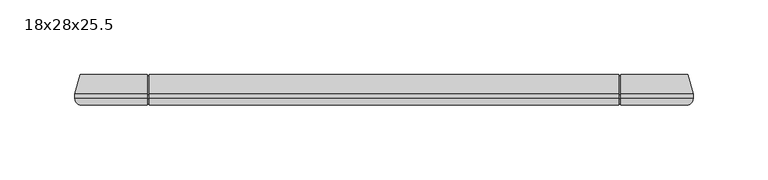
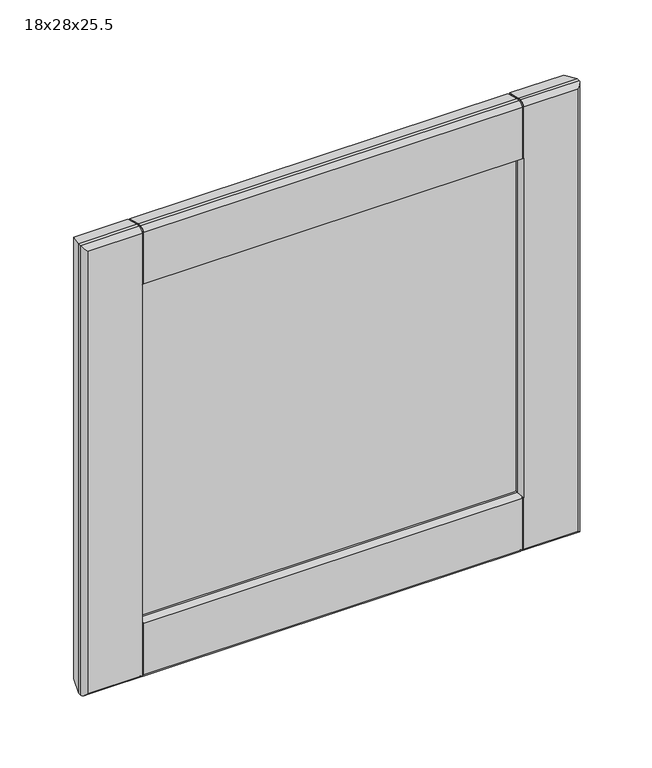
"""IFC4 building model written with IfcOpenShell, lengths in millimetres: furniture geometry, Cabinet-Base-Merillat-Peninsula_Single_Door-Marlin : 18x28x25.5."""

from ifc_helpers import new_model, si_unit, frame, origin, place, context, project, spatial, polyline, circle_curve, ellipse_curve, outline, extrude, source, transform, mapped, element, save
from ifc_brep_helpers import plane_surface, cylinder_surface, advanced_brep


def furniture_18x28x25_5_82de7a22(model_context):
    return source(origin(), model_context, "Body", "SolidModel", [
        advanced_brep(
        [(225.1127049, -696.09335, 63.5), (225.1127049, -696.09335, 457.2), (222.0162124, -700.56375, 454.1035075), (222.0162124, -700.56375, 66.5964925), (225.1127049, -693.32475, 63.5), (225.1127049, -693.32475, 457.2), (221.6075049, -680.24375, 67.0052), (221.6075049, -680.24375, 453.6948), (176.9115422, -680.24375, 111.7011628), (176.5414105, -681.0375, 112.0712945), (174.4602514, -685.50056, 114.1524535), (174.4602514, -685.50056, 406.5475465), (176.5414105, -681.0375, 408.6287055), (176.9115422, -680.24375, 408.9988372), (175.8600209, -687.7406593, 112.752684), (175.8600209, -687.7406593, 407.947316), (190.1877049, -687.99075, 98.425), (190.1877049, -687.99075, 422.275), (190.1877049, -692.81675, 98.425), (190.1877049, -692.81675, 422.275), (175.8600209, -693.0668407, 112.752684), (175.8600209, -693.0668407, 407.947316), (174.4602514, -695.30694, 114.1524535), (174.4602514, -695.30694, 406.5475465), (176.5414105, -699.77, 112.0712945), (176.9086747, -700.5576008, 111.7040302), (176.9115422, -700.56375, 408.9988372), (176.5414105, -699.77, 408.6287055), (-184.5408026, -700.56375, 454.1035075), (-139.4730764, -700.56375, 454.1035075), (-139.4730764, -696.09335, 457.2), (-187.6372951, -696.09335, 457.2), (176.9086747, -696.09335, 457.2), (176.9086747, -700.56375, 454.1035075), (175.3211747, -696.09335, 457.2), (-137.8855764, -696.09335, 457.2), (-137.8855764, -700.56375, 454.1035075), (175.3211747, -700.56375, 454.1035075), (-139.4730764, -693.32475, 457.2), (-187.6372951, -693.32475, 457.2), (176.9086747, -693.32475, 457.2), (175.3211747, -693.32475, 457.2), (-137.8855764, -693.32475, 457.2), (-139.4730764, -680.24375, 453.6948), (-184.1320951, -680.24375, 453.6948), (175.3211747, -680.24375, 453.6948), (-137.8855764, -680.24375, 453.6948), (176.9086747, -680.24375, 453.6948), (-136.9848416, -685.50056, 406.5475465), (-139.0660006, -681.0375, 408.6287055), (-137.8855764, -681.0375, 408.6287055), (-137.8855764, -680.24375, 408.9988372), (175.3211747, -680.24375, 408.9988372), (175.3211747, -681.0375, 408.6287055), (-138.384611, -687.7406593, 407.947316), (-152.7122951, -687.99075, 422.275), (-152.7122951, -692.81675, 422.275), (-138.384611, -693.0668407, 407.947316), (-136.9848416, -695.30694, 406.5475465), (175.3211747, -699.77, 408.6287055), (175.3211747, -700.56375, 408.9988372), (-137.8855764, -700.56375, 408.9988372), (-137.8855764, -699.77, 408.6287055), (-139.0660006, -699.77, 408.6287055), (-187.6372951, -696.09335, 63.5), (-184.5408026, -700.56375, 66.5964925), (-187.6372951, -693.32475, 63.5), (-184.1320951, -680.24375, 67.0052), (-139.4361323, -680.24375, 408.9988372), (-136.9848416, -685.50056, 114.1524535), (-139.0660006, -681.0375, 112.0712945), (-139.4361323, -680.24375, 111.7011628), (-138.384611, -687.7406593, 112.752684), (-152.7122951, -687.99075, 98.425), (-152.7122951, -692.81675, 98.425), (-138.384611, -693.0668407, 112.752684), (-136.9848416, -695.30694, 114.1524535), (-139.4361323, -700.56375, 408.9988372), (-139.4361323, -700.56375, 111.7011628), (-139.0660006, -699.77, 112.0712945), (176.9086747, -700.56375, 66.5964925), (176.9086747, -696.09335, 63.5), (-139.4730764, -696.09335, 63.5), (-139.4730764, -700.56375, 66.5964925), (-137.8855764, -696.09335, 63.5), (175.3211747, -696.09335, 63.5), (175.3211747, -700.56375, 66.5964925), (-137.8855764, -700.56375, 66.5964925), (176.9086747, -693.32475, 63.5), (-139.4730764, -693.32475, 63.5), (-137.8855764, -693.32475, 63.5), (175.3211747, -693.32475, 63.5), (176.9086747, -680.24375, 67.0052), (-139.4730764, -680.24375, 67.0052), (-137.8855764, -680.24375, 67.0052), (175.3211747, -680.24375, 67.0052), (-137.8855764, -680.24375, 111.7011628), (175.3211747, -680.24375, 111.7011628), (175.3211747, -681.0375, 112.0712945), (-137.8855764, -681.0375, 112.0712945), (-137.8855764, -699.77, 112.0712945), (-137.8855764, -700.56375, 111.7011628), (175.3211747, -700.56375, 111.7011628), (175.3211747, -699.77, 112.0712945), (-137.8855764, -699.77, 66.7473948), (-137.8855764, -696.09335, 64.29375), (-137.8855764, -693.4292537, 64.29375), (-137.8855764, -681.0375, 67.6142588), (-139.4730764, -681.0375, 112.0712945), (-139.4730764, -681.0375, 67.6142588), (-139.4730764, -693.4292537, 64.29375), (-139.4730764, -696.09335, 64.29375), (-139.4730764, -699.77, 66.7473948), (-139.4730764, -699.77, 112.0712945), (176.9086747, -699.77, 112.0712945), (176.9086747, -699.77, 66.7473948), (176.9086747, -696.09335, 64.29375), (176.9086747, -693.4292537, 64.29375), (176.9086747, -681.0375, 67.6142588), (176.9086747, -681.0375, 112.0712945), (175.3211747, -681.0375, 67.6142588), (175.3211747, -693.4292537, 64.29375), (175.3211747, -696.09335, 64.29375), (175.3211747, -699.77, 66.7473948), (176.9086747, -681.0375, 408.6287055), (176.9086747, -681.0375, 453.0857412), (176.9086747, -693.4292537, 456.40625), (176.9086747, -696.09335, 456.40625), (176.9086747, -699.77, 453.9526052), (176.9086747, -699.77, 408.6287055), (175.3211747, -699.77, 453.9526052), (175.3211747, -696.09335, 456.40625), (175.3211747, -693.4292537, 456.40625), (175.3211747, -681.0375, 453.0857412), (-137.8855764, -681.0375, 453.0857412), (-137.8855764, -693.4292537, 456.40625), (-137.8855764, -696.09335, 456.40625), (-137.8855764, -699.77, 453.9526052), (-139.4730764, -699.77, 408.6287055), (-139.4730764, -699.77, 453.9526052), (-139.4730764, -696.09335, 456.40625), (-139.4730764, -693.4292537, 456.40625), (-139.4730764, -681.0375, 453.0857412), (-139.4730764, -681.0375, 408.6287055)],
        [
            (0, 1),
            (1, 2, ellipse_curve(frame((220.3375049, -696.09335, 452.4248), z_axis=(0.7071067811865451, 0.0, -0.7071067811865498), x_axis=(-0.7071067811865497, 0.0, -0.7071067811865452)), 6.7531526, 4.7752)),
            (2, 3),
            (3, 0, ellipse_curve(frame((220.3375049, -696.09335, 68.2752), z_axis=(0.7071067811865498, 0.0, 0.7071067811865451), x_axis=(0.7071067811865451, 0.0, -0.70710678118655)), 6.7531526, 4.7752)),
            (0, 4),
            (4, 5),
            (5, 1),
            (4, 6),
            (6, 7),
            (7, 5),
            (8, 9),
            (9, 10),
            (10, 11),
            (11, 12),
            (12, 13),
            (13, 8),
            (10, 14, ellipse_curve(frame((175.8875049, -686.1660992, 112.7252), z_axis=(0.7071067811865498, 0.0, 0.7071067811865451), x_axis=(0.7071067811865451, 0.0, -0.70710678118655)), 2.2271035, 1.5748)),
            (14, 15),
            (15, 11, ellipse_curve(frame((175.8875049, -686.1660992, 407.9748), z_axis=(0.7071067811865451, 0.0, -0.7071067811865498), x_axis=(-0.7071067811865497, 0.0, -0.7071067811865452)), 2.2271035, 1.5748)),
            (14, 16),
            (16, 17),
            (17, 15),
            (16, 18),
            (18, 19),
            (19, 17),
            (18, 20),
            (20, 21),
            (21, 19),
            (20, 22, ellipse_curve(frame((175.8875049, -694.6414008, 112.7252), z_axis=(0.7071067811865498, 0.0, 0.7071067811865451), x_axis=(0.7071067811865451, 0.0, -0.70710678118655)), 2.2271035, 1.5748)),
            (22, 23),
            (23, 21, ellipse_curve(frame((175.8875049, -694.6414008, 407.9748), z_axis=(0.7071067811865451, 0.0, -0.7071067811865498), x_axis=(-0.7071067811865497, 0.0, -0.7071067811865452)), 2.2271035, 1.5748)),
            (22, 24),
            (24, 25),
            (25, 26),
            (26, 27),
            (27, 23),
            (28, 29),
            (29, 30, circle_curve(frame((-139.4730764, -696.09335, 452.4248), z_axis=(-1.0, 0.0, 0.0), x_axis=(0.0, 1.0, 0.0)), 4.7752)),
            (30, 31),
            (31, 28, ellipse_curve(frame((-182.8620951, -696.09335, 452.4248), z_axis=(0.7071067811865498, 0.0, 0.7071067811865451), x_axis=(0.7071067811865452, 0.0, -0.7071067811865497)), 6.7531526, 4.7752)),
            (1, 32),
            (32, 33, circle_curve(frame((176.9086747, -696.09335, 452.4248), z_axis=(1.0, 0.0, 0.0), x_axis=(0.0, 1.0, 0.0)), 4.7752)),
            (33, 2),
            (34, 35),
            (35, 36, circle_curve(frame((-137.8855764, -696.09335, 452.4248), z_axis=(1.0, 0.0, 0.0), x_axis=(0.0, 1.0, 0.0)), 4.7752)),
            (36, 37),
            (37, 34, circle_curve(frame((175.3211747, -696.09335, 452.4248), z_axis=(-1.0, 0.0, 0.0), x_axis=(0.0, 1.0, 0.0)), 4.7752)),
            (30, 38),
            (38, 39),
            (39, 31),
            (5, 40),
            (40, 32),
            (41, 42),
            (42, 35),
            (34, 41),
            (38, 43),
            (43, 44),
            (44, 39),
            (45, 46),
            (46, 42),
            (41, 45),
            (7, 47),
            (47, 40),
            (48, 49),
            (49, 50),
            (50, 51),
            (51, 52),
            (52, 53),
            (53, 12),
            (11, 48),
            (15, 54),
            (54, 48, ellipse_curve(frame((-138.4120951, -686.1660992, 407.9748), z_axis=(0.7071067811865498, 0.0, 0.7071067811865451), x_axis=(0.7071067811865452, 0.0, -0.7071067811865497)), 2.2271035, 1.5748)),
            (17, 55),
            (55, 54),
            (19, 56),
            (56, 55),
            (21, 57),
            (57, 56),
            (23, 58),
            (58, 57, ellipse_curve(frame((-138.4120951, -694.6414008, 407.9748), z_axis=(0.7071067811865498, 0.0, 0.7071067811865451), x_axis=(0.7071067811865452, 0.0, -0.7071067811865497)), 2.2271035, 1.5748)),
            (27, 59),
            (59, 60),
            (60, 61),
            (61, 62),
            (62, 63),
            (63, 58),
            (31, 64),
            (64, 65, ellipse_curve(frame((-182.8620951, -696.09335, 68.2752), z_axis=(-0.7071067811865451, 0.0, 0.7071067811865498), x_axis=(0.7071067811865497, 0.0, 0.7071067811865452)), 6.7531526, 4.7752)),
            (65, 28),
            (39, 66),
            (66, 64),
            (44, 67),
            (67, 66),
            (68, 49),
            (48, 69),
            (69, 70),
            (70, 71),
            (71, 68),
            (54, 72),
            (72, 69, ellipse_curve(frame((-138.4120951, -686.1660992, 112.7252), z_axis=(-0.7071067811865451, 0.0, 0.7071067811865498), x_axis=(0.7071067811865497, 0.0, 0.7071067811865452)), 2.2271035, 1.5748)),
            (55, 73),
            (73, 72),
            (56, 74),
            (74, 73),
            (57, 75),
            (75, 74),
            (58, 76),
            (76, 75, ellipse_curve(frame((-138.4120951, -694.6414008, 112.7252), z_axis=(-0.7071067811865451, 0.0, 0.7071067811865498), x_axis=(0.7071067811865497, 0.0, 0.7071067811865452)), 2.2271035, 1.5748)),
            (63, 77),
            (77, 78),
            (78, 79),
            (79, 76),
            (3, 80),
            (80, 81, circle_curve(frame((176.9086747, -696.09335, 68.2752), z_axis=(1.0, 0.0, 0.0), x_axis=(0.0, 1.0, 0.0)), 4.7752)),
            (81, 0),
            (64, 82),
            (82, 83, circle_curve(frame((-139.4730764, -696.09335, 68.2752), z_axis=(-1.0, 0.0, 0.0), x_axis=(0.0, 1.0, 0.0)), 4.7752)),
            (83, 65),
            (84, 85),
            (85, 86, circle_curve(frame((175.3211747, -696.09335, 68.2752), z_axis=(-1.0, 0.0, 0.0), x_axis=(0.0, 1.0, 0.0)), 4.7752)),
            (86, 87),
            (87, 84, circle_curve(frame((-137.8855764, -696.09335, 68.2752), z_axis=(1.0, 0.0, 0.0), x_axis=(0.0, 1.0, 0.0)), 4.7752)),
            (81, 88),
            (88, 4),
            (66, 89),
            (89, 82),
            (90, 91),
            (91, 85),
            (84, 90),
            (88, 92),
            (92, 6),
            (67, 93),
            (93, 89),
            (94, 95),
            (95, 91),
            (90, 94),
            (51, 46),
            (45, 52),
            (43, 68),
            (71, 93),
            (92, 8),
            (13, 47),
            (96, 97),
            (97, 95),
            (94, 96),
            (9, 98),
            (98, 97),
            (96, 99),
            (99, 70),
            (69, 10),
            (72, 14),
            (73, 16),
            (74, 18),
            (75, 20),
            (76, 22),
            (79, 100),
            (100, 101),
            (101, 102),
            (102, 103),
            (103, 24),
            (33, 26),
            (25, 80),
            (36, 61),
            (60, 37),
            (83, 78),
            (77, 29),
            (86, 102),
            (101, 87),
            (100, 104),
            (104, 105, circle_curve(frame((-137.8855764, -696.09335, 68.2752), z_axis=(1.0, 0.0, 0.0), x_axis=(0.0, 0.0, -1.0)), 3.98145)),
            (105, 106),
            (106, 107),
            (107, 99),
            (71, 108),
            (108, 109),
            (109, 110),
            (110, 111),
            (111, 112, circle_curve(frame((-139.4730764, -696.09335, 68.2752), z_axis=(-1.0, 0.0, 0.0), x_axis=(0.0, 0.0, -1.0)), 3.98145)),
            (112, 113),
            (113, 78),
            (113, 79),
            (112, 104),
            (111, 105),
            (110, 106),
            (109, 107),
            (108, 70),
            (25, 114),
            (114, 115),
            (115, 116, circle_curve(frame((176.9086747, -696.09335, 68.2752), z_axis=(1.0, 0.0, 0.0), x_axis=(0.0, 0.0, -1.0)), 3.98145)),
            (116, 117),
            (117, 118),
            (118, 119),
            (119, 8),
            (98, 120),
            (120, 121),
            (121, 122),
            (122, 123, circle_curve(frame((175.3211747, -696.09335, 68.2752), z_axis=(-1.0, 0.0, 0.0), x_axis=(0.0, 0.0, -1.0)), 3.98145)),
            (123, 103),
            (24, 114),
            (123, 115),
            (122, 116),
            (121, 117),
            (120, 118),
            (9, 119),
            (13, 124),
            (124, 125),
            (125, 126),
            (126, 127),
            (127, 128, circle_curve(frame((176.9086747, -696.09335, 452.4248), z_axis=(1.0, 0.0, 0.0), x_axis=(0.0, 0.0, -1.0)), 3.98145)),
            (128, 129),
            (129, 26),
            (59, 130),
            (130, 131, circle_curve(frame((175.3211747, -696.09335, 452.4248), z_axis=(-1.0, 0.0, 0.0), x_axis=(0.0, 0.0, -1.0)), 3.98145)),
            (131, 132),
            (132, 133),
            (133, 53),
            (12, 124),
            (133, 125),
            (132, 126),
            (131, 127),
            (130, 128),
            (27, 129),
            (50, 134),
            (134, 135),
            (135, 136),
            (136, 137, circle_curve(frame((-137.8855764, -696.09335, 452.4248), z_axis=(1.0, 0.0, 0.0), x_axis=(0.0, 0.0, -1.0)), 3.98145)),
            (137, 62),
            (138, 139),
            (139, 140, circle_curve(frame((-139.4730764, -696.09335, 452.4248), z_axis=(-1.0, 0.0, 0.0), x_axis=(0.0, 0.0, -1.0)), 3.98145)),
            (140, 141),
            (141, 142),
            (142, 143),
            (143, 68),
            (77, 138),
            (63, 138),
            (143, 49),
            (142, 134),
            (141, 135),
            (140, 136),
            (139, 137),
        ],
        [
            cylinder_surface(frame((220.3375049, -696.09335, 63.5), z_axis=(0.0, 0.0, -1.0), x_axis=(0.0, 1.0, 0.0)), 4.7752),
            plane_surface(frame((225.1127049, -696.09335, 63.5), z_axis=(1.0, 0.0, 0.0), x_axis=(0.0, 0.0, 1.0))),
            plane_surface(frame((225.1127049, -693.32475, 63.5), z_axis=(0.9659229350723619, 0.25882983502910506, 0.0), x_axis=(0.0, 0.0, 1.0))),
            plane_surface(frame((176.9115422, -680.24375, 111.7011628), z_axis=(-0.9063077870366099, 0.4226182617407856, 0.0), x_axis=(0.0, 0.0, 1.0))),
            cylinder_surface(frame((175.8875049, -686.1660992, 63.5), z_axis=(0.0, 0.0, -1.0000000000000002), x_axis=(-0.01745240643729364, -0.9998476951563912, 0.0)), 1.5748),
            plane_surface(frame((175.8600209, -687.7406593, 112.752684), z_axis=(-0.017452406437322144, -0.9998476951563906, 0.0), x_axis=(0.0, 0.0, 1.0))),
            plane_surface(frame((190.1877049, -687.99075, 98.425), z_axis=(-1.0, 0.0, 0.0), x_axis=(0.0, 0.0, 1.0))),
            plane_surface(frame((190.1877049, -692.81675, 98.425), z_axis=(-0.01745240643727848, 0.9998476951563914, 0.0), x_axis=(0.0, 0.0, 1.0))),
            cylinder_surface(frame((175.8875049, -694.6414008, 63.5), z_axis=(0.0, 0.0, -1.0000000000000002), x_axis=(-0.9063077870367326, -0.42261826174052236, 0.0)), 1.5748),
            plane_surface(frame((174.4602514, -695.30694, 114.1524535), z_axis=(-0.9063077870366333, -0.4226182617407352, 0.0), x_axis=(0.0, 0.0, 1.0))),
            cylinder_surface(frame((225.1127049, -696.09335, 452.4248), z_axis=(1.0, 0.0, 0.0), x_axis=(0.0, 1.0, 0.0)), 4.7752),
            plane_surface(frame((225.1127049, -696.09335, 457.2), z_axis=(0.0, 0.0, 1.0), x_axis=(-1.0, 0.0, 0.0))),
            plane_surface(frame((225.1127049, -693.32475, 457.2), z_axis=(0.0, 0.25882983502910506, 0.9659229350723619), x_axis=(-1.0, 0.0, 0.0))),
            plane_surface(frame((176.9115422, -680.24375, 408.9988372), z_axis=(0.0, 0.4226182617407856, -0.9063077870366099), x_axis=(-1.0, 0.0, 0.0))),
            cylinder_surface(frame((225.1127049, -686.1660992, 407.9748), z_axis=(1.0000000000000002, 0.0, 0.0), x_axis=(0.0, -0.9998476951563912, -0.01745240643729364)), 1.5748),
            plane_surface(frame((175.8600209, -687.7406593, 407.947316), z_axis=(0.0, -0.9998476951563906, -0.017452406437322144), x_axis=(-1.0, 0.0, 0.0))),
            plane_surface(frame((190.1877049, -687.99075, 422.275), z_axis=(0.0, 0.0, -1.0), x_axis=(-1.0, 0.0, 0.0))),
            plane_surface(frame((190.1877049, -692.81675, 422.275), z_axis=(0.0, 0.9998476951563914, -0.01745240643727848), x_axis=(-1.0, 0.0, 0.0))),
            cylinder_surface(frame((225.1127049, -694.6414008, 407.9748), z_axis=(1.0000000000000002, 0.0, 0.0), x_axis=(0.0, -0.42261826174052236, -0.9063077870367326)), 1.5748),
            plane_surface(frame((174.4602514, -695.30694, 406.5475465), z_axis=(0.0, -0.4226182617407352, -0.9063077870366333), x_axis=(-1.0, 0.0, 0.0))),
            cylinder_surface(frame((-182.8620951, -696.09335, 457.2), z_axis=(0.0, 0.0, 1.0), x_axis=(0.0, 1.0, 0.0)), 4.7752),
            plane_surface(frame((-187.6372951, -696.09335, 457.2), z_axis=(-1.0, 0.0, 0.0), x_axis=(0.0, 0.0, -1.0))),
            plane_surface(frame((-187.6372951, -693.32475, 457.2), z_axis=(-0.9659229350723619, 0.25882983502910506, 0.0), x_axis=(0.0, 0.0, -1.0))),
            plane_surface(frame((-139.4361323, -680.24375, 408.9988372), z_axis=(0.9063077870366099, 0.4226182617407856, 0.0), x_axis=(0.0, 0.0, -1.0))),
            cylinder_surface(frame((-138.4120951, -686.1660992, 457.2), z_axis=(0.0, 0.0, 1.0000000000000002), x_axis=(0.01745240643729364, -0.9998476951563912, 0.0)), 1.5748),
            plane_surface(frame((-138.384611, -687.7406593, 407.947316), z_axis=(0.017452406437322144, -0.9998476951563906, 0.0), x_axis=(0.0, 0.0, -1.0))),
            plane_surface(frame((-152.7122951, -687.99075, 422.275), z_axis=(1.0, 0.0, 0.0), x_axis=(0.0, 0.0, -1.0))),
            plane_surface(frame((-152.7122951, -692.81675, 422.275), z_axis=(0.01745240643727848, 0.9998476951563914, 0.0), x_axis=(0.0, 0.0, -1.0))),
            cylinder_surface(frame((-138.4120951, -694.6414008, 457.2), z_axis=(0.0, 0.0, 1.0000000000000002), x_axis=(0.9063077870367326, -0.42261826174052236, 0.0)), 1.5748),
            plane_surface(frame((-136.9848416, -695.30694, 406.5475465), z_axis=(0.9063077870366333, -0.4226182617407352, 0.0), x_axis=(0.0, 0.0, -1.0))),
            cylinder_surface(frame((-187.6372951, -696.09335, 68.2752), z_axis=(-1.0, 0.0, 0.0), x_axis=(0.0, 1.0, 0.0)), 4.7752),
            plane_surface(frame((-187.6372951, -696.09335, 63.5), z_axis=(0.0, 0.0, -1.0), x_axis=(1.0, 0.0, 0.0))),
            plane_surface(frame((-187.6372951, -693.32475, 63.5), z_axis=(0.0, 0.25882983502910506, -0.9659229350723619), x_axis=(1.0, 0.0, 0.0))),
            plane_surface(frame((-184.1320951, -680.24375, 67.0052), z_axis=(0.0, 1.0, 0.0), x_axis=(1.0, 0.0, 0.0))),
            plane_surface(frame((-139.4361323, -680.24375, 111.7011628), z_axis=(0.0, 0.4226182617407856, 0.9063077870366099), x_axis=(1.0, 0.0, 0.0))),
            cylinder_surface(frame((-187.6372951, -686.1660992, 112.7252), z_axis=(-1.0000000000000002, 0.0, 0.0), x_axis=(0.0, -0.9998476951563912, 0.01745240643729364)), 1.5748),
            plane_surface(frame((-138.384611, -687.7406593, 112.752684), z_axis=(0.0, -0.9998476951563906, 0.017452406437322144), x_axis=(1.0, 0.0, 0.0))),
            plane_surface(frame((-152.7122951, -687.99075, 98.425), z_axis=(0.0, 0.0, 1.0), x_axis=(1.0, 0.0, 0.0))),
            plane_surface(frame((-152.7122951, -692.81675, 98.425), z_axis=(0.0, 0.9998476951563914, 0.01745240643727848), x_axis=(1.0, 0.0, 0.0))),
            cylinder_surface(frame((-187.6372951, -694.6414008, 112.7252), z_axis=(-1.0000000000000002, 0.0, 0.0), x_axis=(0.0, -0.42261826174052236, 0.9063077870367326)), 1.5748),
            plane_surface(frame((-136.9848416, -695.30694, 114.1524535), z_axis=(0.0, -0.4226182617407352, 0.9063077870366333), x_axis=(1.0, 0.0, 0.0))),
            plane_surface(frame((-139.4361323, -700.56375, 111.7011628), z_axis=(0.0, -1.0, 0.0), x_axis=(1.0, 0.0, 0.0))),
            plane_surface(frame((-137.8855764, -700.56375, 111.7011628), z_axis=(-1.0000000000000002, 0.0, 0.0), x_axis=(0.0, 0.9063077870366303, 0.4226182617407418))),
            plane_surface(frame((-139.4730764, -700.56375, 111.7011628), z_axis=(1.0000000000000002, 0.0, 0.0), x_axis=(0.0, -0.9063077870366303, -0.4226182617407418))),
            plane_surface(frame((-137.8855764, -700.56375, 111.7011628), z_axis=(0.0, 0.4226182617407418, -0.9063077870366303), x_axis=(-1.0, 0.0, 0.0))),
            plane_surface(frame((-137.8855764, -699.77, 112.0712945), z_axis=(0.0, -1.0, 0.0), x_axis=(-1.0, 0.0, 0.0))),
            cylinder_surface(frame((-139.4730764, -696.09335, 68.2752), z_axis=(-1.0, 0.0, 0.0), x_axis=(0.0, 0.0, -1.0)), 3.98145),
            plane_surface(frame((-137.8855764, -696.09335, 64.29375), z_axis=(0.0, 0.0, -1.0), x_axis=(-1.0, 0.0, 0.0))),
            plane_surface(frame((-137.8855764, -693.4292537, 64.29375), z_axis=(0.0, 0.25882983502916795, -0.9659229350723451), x_axis=(-1.0, 0.0, 0.0))),
            plane_surface(frame((-137.8855764, -681.0375, 67.6142588), z_axis=(0.0, 1.0, 0.0), x_axis=(-1.0, 0.0, 0.0))),
            plane_surface(frame((-137.8855764, -681.0375, 112.0712945), z_axis=(0.0, -0.4226182617407951, -0.9063077870366054), x_axis=(-1.0, 0.0, 0.0))),
            plane_surface(frame((176.9086747, -700.56375, 111.7011628), z_axis=(-1.0, 0.0, 0.0), x_axis=(0.0, 0.9063077870366284, 0.42261826174074574))),
            plane_surface(frame((175.3211747, -700.56375, 111.7011628), z_axis=(1.0, 0.0, 0.0), x_axis=(0.0, -0.9063077870366284, -0.42261826174074574))),
            plane_surface(frame((176.9086747, -700.56375, 111.7011628), z_axis=(0.0, 0.42261826174074574, -0.9063077870366284), x_axis=(-1.0, 0.0, 0.0))),
            plane_surface(frame((176.9086747, -699.77, 112.0712945), z_axis=(0.0, -1.0, 0.0), x_axis=(-1.0, 0.0, 0.0))),
            cylinder_surface(frame((175.3211747, -696.09335, 68.2752), z_axis=(-1.0, 0.0, 0.0), x_axis=(0.0, 0.0, -1.0)), 3.98145),
            plane_surface(frame((176.9086747, -696.09335, 64.29375), z_axis=(0.0, 0.0, -1.0), x_axis=(-1.0, 0.0, 0.0))),
            plane_surface(frame((176.9086747, -693.4292537, 64.29375), z_axis=(0.0, 0.25882983502917023, -0.9659229350723445), x_axis=(-1.0, 0.0, 0.0))),
            plane_surface(frame((176.9086747, -681.0375, 67.6142588), z_axis=(0.0, 1.0, 0.0), x_axis=(-1.0, 0.0, 0.0))),
            plane_surface(frame((176.9086747, -681.0375, 112.0712945), z_axis=(0.0, -0.4226182617408056, -0.9063077870366005), x_axis=(-1.0, 0.0, 0.0))),
            plane_surface(frame((176.9086747, -696.09335, 447.6496), z_axis=(-1.0, 0.0, 0.0), x_axis=(0.0, -1.0, 0.0))),
            plane_surface(frame((175.3211747, -696.09335, 447.6496), z_axis=(1.0, 0.0, 0.0), x_axis=(0.0, 1.0, 0.0))),
            plane_surface(frame((176.9086747, -680.24375, 408.9988372), z_axis=(0.0, -0.4226182617407918, 0.906307787036607), x_axis=(-1.0, 0.0, 0.0))),
            plane_surface(frame((176.9086747, -681.0375, 408.6287055), z_axis=(0.0, 1.0, 0.0), x_axis=(-1.0, 0.0, 0.0))),
            plane_surface(frame((176.9086747, -681.0375, 453.0857412), z_axis=(0.0, 0.25882983502943885, 0.9659229350722724), x_axis=(-1.0, 0.0, 0.0))),
            plane_surface(frame((176.9086747, -693.4292537, 456.40625), z_axis=(0.0, 0.0, 1.0), x_axis=(-1.0, 0.0, 0.0))),
            cylinder_surface(frame((175.3211747, -696.09335, 452.4248), z_axis=(-1.0, 0.0, 0.0), x_axis=(0.0, 0.0, -1.0)), 3.98145),
            plane_surface(frame((176.9086747, -699.77, 453.9526052), z_axis=(0.0, -1.0, 0.0), x_axis=(-1.0, 0.0, 0.0))),
            plane_surface(frame((176.9086747, -699.77, 408.6287055), z_axis=(0.0, 0.42261826174073464, 0.9063077870366336), x_axis=(-1.0, 0.0, 0.0))),
            plane_surface(frame((-137.8855764, -699.77, 408.6287055), z_axis=(-1.0, 0.0, 0.0), x_axis=(0.0, -0.9063077870366311, 0.4226182617407399))),
            plane_surface(frame((-139.4730764, -699.77, 408.6287055), z_axis=(1.0, 0.0, 0.0), x_axis=(0.0, 0.9063077870366311, -0.4226182617407399))),
            plane_surface(frame((-137.8855764, -699.77, 408.6287055), z_axis=(0.0, 0.4226182617407399, 0.9063077870366311), x_axis=(-1.0, 0.0, 0.0))),
            plane_surface(frame((-137.8855764, -680.24375, 408.9988372), z_axis=(0.0, -0.42261826174079353, 0.9063077870366061), x_axis=(-1.0, 0.0, 0.0))),
            plane_surface(frame((-137.8855764, -681.0375, 408.6287055), z_axis=(0.0, 1.0, 0.0), x_axis=(-1.0, 0.0, 0.0))),
            plane_surface(frame((-137.8855764, -681.0375, 453.0857412), z_axis=(0.0, 0.2588298350294384, 0.9659229350722726), x_axis=(-1.0, 0.0, 0.0))),
            plane_surface(frame((-137.8855764, -693.4292537, 456.40625), z_axis=(0.0, 0.0, 1.0), x_axis=(-1.0, 0.0, 0.0))),
            cylinder_surface(frame((-139.4730764, -696.09335, 452.4248), z_axis=(-1.0, 0.0, 0.0), x_axis=(0.0, 0.0, -1.0)), 3.98145),
            plane_surface(frame((-137.8855764, -699.77, 453.9526052), z_axis=(0.0, -1.0, 0.0), x_axis=(-1.0, 0.0, 0.0))),
        ],
        [
            (0, [[1, 2, 3, 4]]),
            (1, [[5, 6, 7, -1]]),
            (2, [[8, 9, 10, -6]]),
            (3, [[11, 12, 13, 14, 15, 16]]),
            (4, [[17, 18, 19, -13]]),
            (5, [[20, 21, 22, -18]]),
            (6, [[23, 24, 25, -21]]),
            (7, [[26, 27, 28, -24]]),
            (8, [[29, 30, 31, -27]]),
            (9, [[32, 33, 34, 35, 36, -30]]),
            (10, [[37, 38, 39, 40]]),
            (10, [[41, 42, 43, -2]]),
            (10, [[44, 45, 46, 47]]),
            (11, [[-39, 48, 49, 50]]),
            (11, [[51, 52, -41, -7]]),
            (11, [[53, 54, -44, 55]]),
            (12, [[-49, 56, 57, 58]]),
            (12, [[59, 60, -53, 61]]),
            (12, [[62, 63, -51, -10]]),
            (13, [[64, 65, 66, 67, 68, 69, -14, 70]]),
            (14, [[71, 72, -70, -19]]),
            (15, [[73, 74, -71, -22]]),
            (16, [[75, 76, -73, -25]]),
            (17, [[77, 78, -75, -28]]),
            (18, [[79, 80, -77, -31]]),
            (19, [[-36, 81, 82, 83, 84, 85, 86, -79]]),
            (20, [[87, 88, 89, -40]]),
            (21, [[90, 91, -87, -50]]),
            (22, [[92, 93, -90, -58]]),
            (23, [[94, -64, 95, 96, 97, 98]]),
            (24, [[99, 100, -95, -72]]),
            (25, [[101, 102, -99, -74]]),
            (26, [[103, 104, -101, -76]]),
            (27, [[105, 106, -103, -78]]),
            (28, [[107, 108, -105, -80]]),
            (29, [[-86, 109, 110, 111, 112, -107]]),
            (30, [[113, 114, 115, -4]]),
            (30, [[116, 117, 118, -88]]),
            (30, [[119, 120, 121, 122]]),
            (31, [[-115, 123, 124, -5]]),
            (31, [[125, 126, -116, -91]]),
            (31, [[127, 128, -119, 129]]),
            (32, [[-124, 130, 131, -8]]),
            (32, [[132, 133, -125, -93]]),
            (32, [[134, 135, -127, 136]]),
            (33, [[-67, 137, -59, 138]]),
            (33, [[-57, 139, -98, 140, -132, -92]]),
            (33, [[-131, 141, -16, 142, -62, -9]]),
            (33, [[143, 144, -134, 145]]),
            (34, [[-12, 146, 147, -143, 148, 149, -96, 150]]),
            (35, [[-150, -100, 151, -17]]),
            (36, [[-151, -102, 152, -20]]),
            (37, [[-152, -104, 153, -23]]),
            (38, [[-153, -106, 154, -26]]),
            (39, [[-154, -108, 155, -29]]),
            (40, [[-112, 156, 157, 158, 159, 160, -32, -155]]),
            (41, [[-43, 161, -34, 162, -113, -3]]),
            (41, [[-46, 163, -83, 164]]),
            (41, [[-118, 165, -110, 166, -37, -89]]),
            (41, [[-121, 167, -158, 168]]),
            (42, [[-148, -145, -136, -129, -122, -168, -157, 169, 170, 171, 172, 173]]),
            (43, [[-165, -117, -126, -133, -140, 174, 175, 176, 177, 178, 179, 180]]),
            (44, [[181, -111, -180]]),
            (45, [[-156, -181, -179, 182, -169]]),
            (46, [[-182, -178, 183, -170]]),
            (47, [[-183, -177, 184, -171]]),
            (48, [[-184, -176, 185, -172]]),
            (49, [[-185, -175, 186, -149, -173]]),
            (50, [[-97, -186, -174]]),
            (51, [[-141, -130, -123, -114, -162, 187, 188, 189, 190, 191, 192, 193]]),
            (52, [[-159, -167, -120, -128, -135, -144, -147, 194, 195, 196, 197, 198]]),
            (53, [[-33, 199, -187]]),
            (54, [[-199, -160, -198, 200, -188]]),
            (55, [[-200, -197, 201, -189]]),
            (56, [[-201, -196, 202, -190]]),
            (57, [[-202, -195, 203, -191]]),
            (58, [[-203, -194, -146, 204, -192]]),
            (59, [[-204, -11, -193]]),
            (60, [[-161, -42, -52, -63, -142, 205, 206, 207, 208, 209, 210, 211]]),
            (61, [[-68, -138, -61, -55, -47, -164, -82, 212, 213, 214, 215, 216]]),
            (62, [[-15, 217, -205]]),
            (63, [[-217, -69, -216, 218, -206]]),
            (64, [[-218, -215, 219, -207]]),
            (65, [[-219, -214, 220, -208]]),
            (66, [[-220, -213, 221, -209]]),
            (67, [[-221, -212, -81, 222, -210]]),
            (68, [[-222, -35, -211]]),
            (69, [[-84, -163, -45, -54, -60, -137, -66, 223, 224, 225, 226, 227]]),
            (70, [[228, 229, 230, 231, 232, 233, -139, -56, -48, -38, -166, 234]]),
            (71, [[-109, 235, -234]]),
            (72, [[236, -94, -233]]),
            (73, [[-65, -236, -232, 237, -223]]),
            (74, [[-237, -231, 238, -224]]),
            (75, [[-238, -230, 239, -225]]),
            (76, [[-239, -229, 240, -226]]),
            (77, [[-240, -228, -235, -85, -227]]),
        ],
    ),
        extrude(outline(polyline([(-152.7122951, -692.81675), (-152.7122951, -687.99075), (190.1877049, -687.99075), (190.1877049, -692.81675), (-152.7122951, -692.81675)])), frame((0.0, 0.0, 98.425), z_axis=(0.0, 0.0, 1.0), x_axis=(1.0, 0.0, 0.0)), (0.0, 0.0, 1.0), 323.85),
    ])


if __name__ == "__main__":
    model = new_model("IFC4")
    model_context = context("Model", 3, world=origin())
    ifc_project = project(units=[si_unit("LENGTHUNIT", "METRE", prefix="MILLI")], contexts=[model_context])
    site = spatial("IfcSite", under=ifc_project)
    building = spatial("IfcBuilding", under=site)
    placement = place(None, origin())
    furniture_18x28x25_5_shape = furniture_18x28x25_5_82de7a22(model_context)
    element("IfcFurniture", 1, ObjectType="Cabinet-Base-Merillat-Peninsula_Single_Door-Marlin : 18x28x25.5", at=placement, inside=building, context=model_context, shape_type="MappedRepresentation", body=[
        mapped(furniture_18x28x25_5_shape, transform((0.0, 0.0, 0.0), x_axis=(1.0, 0.0, 0.0), y_axis=(0.0, 1.0, 0.0), z_axis=(0.0, 0.0, 1.0))),
    ])
    save(model, "model.ifc")

# Revit data of these elements
# Type "Cabinet-Base-Merillat-Peninsula_Single_Door-Marlin : 18x28x25.5"
#   URL = "http://www.merillat.com"
#   Toe Kick Note = "Toe Kick Covering is not included. To be purchased Separately."
#   Product Page URL = "http://www.merillat.com//our-products/rooms/kitchen/"
#   Product Line = "Express"
#   Product Group = "Base Cabinet"
#   Product Documentation Link = "http://merillatbusiness.com/customer-resources/product-line-resources/merillat-classic/"
#   Model = "PB18"
#   Manufacturer = "Merillat"
#   Finish = "Wood"
#   Description = "Peninsula Base Single Door"
#   Construction Type = "Peninsula Base Single Door"
#   Cabinet Construction Note = "One standard height full width drawer opens on kitchen side, peninsula side has one full width drawer front above door, door hinged left on kitchen side, FDS option or tray option must be selected for this cabinet"
#   Assembly Code = "C1030410"
#   Top and Bottom Spacing = 0' - 1"
#   Toe Kick Height = 0' - 1 1/2"
#   Toe Kick Depth = 0' - 2 25/32"
#   Depth = 2' - 4 7/32"
#   Height = 2' - 1 1/2"
#   Width = 1' - 6"
#   Cabinet Shell = 0' - 0 3/8"
#   Cabinet Drawer Width = 1' - 4 1/4"
#   Cabinet Drawer Height = 0' - 5 1/2"
#   Cabinet Door Width = 1' - 4 1/4"
#   Cabinet Door Height = 1' - 3 1/2"
#   COBie.Type = no
#   Partial Overlay = yes
#   Full Overlay = no
#   Elevation Swing Line = yes
#   Toe Kick Material = Wood - Merillat - Raw Particle Board
#   Door Drawer Material = Wood - Merillat - Pecan(1)
#   Cabinet Material = Wood - Merillat - Pecan(1)
#   Cabinet Drawer Style = element 802166
#   Cabinet Door Style = element 802165
# Element 1 (IfcFurniture, "Cabinet-Base-Merillat-Peninsula_Single_Door-Marlin : 18x28x25.5")
#   Materials on its faces: "Wood - Merillat - Pecan(1)", "Wood - Merillat - Raw Particle Board"
# Materials
#   "Wood - Merillat - Raw Particle Board": class "Plastic", colour RGB 80 80 80, transparency 0, Description = "Plastic Laminate - Navy", Cost = 0
#   "Wood - Merillat - Pecan(1)": class "Wood", colour RGB 108 67 43, transparency 0, Cost = 0
